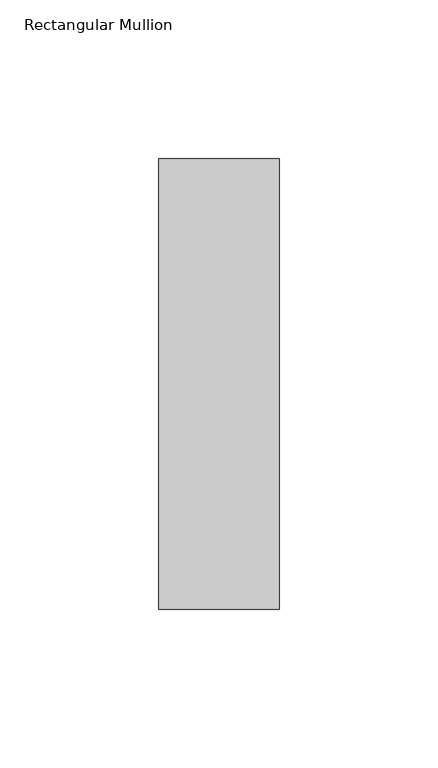
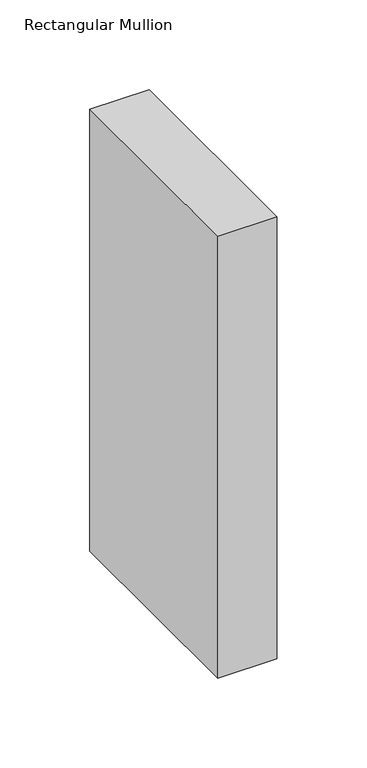
"""IFC4 building model written with IfcOpenShell, lengths in millimetres: member geometry, Rectangular Mullion : NLRS_21_CWM_hsb-regel 38x142_gen_rsf."""

from ifc_helpers import new_model, si_unit, frame, origin, place, context, project, spatial, polyline, outline, extrude, source, transform, mapped, element, save


def rectangular_mullion_25b390b2(model_context):
    return source(origin(), model_context, "Body", "SweptSolid", [
        extrude(outline(polyline([(-38.0, -71.0), (-38.0, 71.0), (0.0, 71.0), (0.0, -71.0), (-38.0, -71.0)])), frame((0.0, 0.0, -300.0), z_axis=(0.0, 0.0, 1.0), x_axis=(1.0, 0.0, 0.0)), (0.0, 0.0, 1.0), 300.0),
    ])


if __name__ == "__main__":
    model = new_model("IFC4")
    model_context = context("Model", 3, world=origin())
    ifc_project = project(units=[si_unit("LENGTHUNIT", "METRE", prefix="MILLI")], contexts=[model_context])
    site = spatial("IfcSite", under=ifc_project)
    building = spatial("IfcBuilding", under=site)
    placement = place(None, origin())
    rectangular_mullion_shape = rectangular_mullion_25b390b2(model_context)
    element("IfcMember", 1, ObjectType="Rectangular Mullion : NLRS_21_CWM_hsb-regel 38x142_gen_rsf", at=placement, inside=building, context=model_context, shape_type="MappedRepresentation", body=[
        mapped(rectangular_mullion_shape, transform((0.0, 0.0, 0.0), x_axis=(1.0, 0.0, 0.0), y_axis=(0.0, 1.0, 0.0), z_axis=(0.0, 0.0, 1.0))),
    ])
    save(model, "model.ifc")

# Revit data of these elements
# Type "Rectangular Mullion : NLRS_21_CWM_hsb-regel 38x142_gen_rsf"
#   Export Type to IFC As = "IfcWall"
#   Type IfcGUID = "07M7mRoiH1CR8m_RSKIwpF"
#   Assembly Code = "21.10"
#   built-in parameter 1007322 = 0.465879 (stored number, unit not read)
#   built-in parameter 1007321 = 0.062336 (stored number, unit not read)
#   built-in parameter 1007320 = 0.062336 (stored number, unit not read)
# Element 1 (IfcMember, "Rectangular Mullion : NLRS_21_CWM_hsb-regel 38x142_gen_rsf")
#   Materials on its faces: "NLRS_i2_hout naaldhout vuren_gen_rsf"
# Materials
#   "NLRS_i2_hout naaldhout vuren_gen_rsf": class "I - Hout", colour RGB 234 199 147, transparency 0, Keynote = "i2", Manufacturer = "Revit Standards Foundation", URL = "www.revitstandards.org", Description = "hout vuren", Cost = 0
